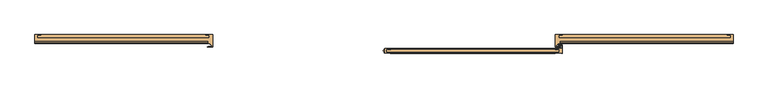
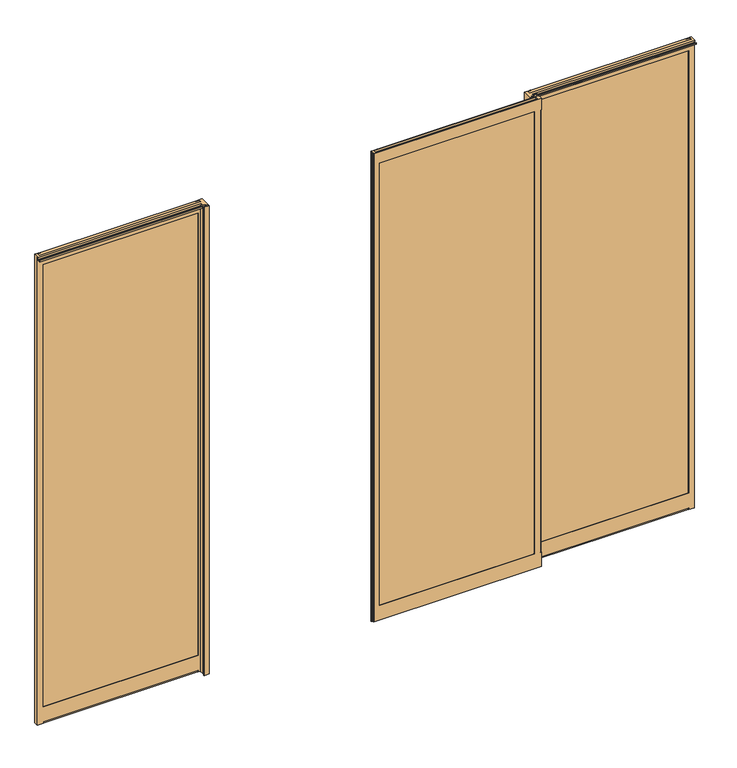
"""IFC4 building model written with IfcOpenShell, lengths in millimetres: door geometry, Otomatik Kapı-Çift Kanat : Otomatik Kapı - Çift Kanat - 150-220."""

from ifc_helpers import new_model, si_unit, point, frame, frame_2d, origin, place, context, project, spatial, polyline, circle_curve, trimmed, segment, composite_curve, outline, extrude, source, transform, mapped, element, save
from ifc_brep_helpers import plane_surface, cylinder_surface, revolved_surface, advanced_brep


def door_0aad8b15(model_context):
    return source(origin(), model_context, "Body", "SolidModel", [
        advanced_brep(
        [(1455.0015, 82.5, 0.0), (1480.0, 82.5, 0.0), (1480.0, 62.5, 0.0), (1455.0015331, 62.5, 0.0), (1455.0015331, 64.5000235, 0.0), (755.8014669, 64.5000827, 0.0), (755.8014669, 62.5, 0.0), (745.7999735, 62.5, 0.0), (745.7999735, 44.6000769, 0.0), (735.7999977, 44.6000769, 0.0), (735.7999977, 41.4071569, 0.0), (730.5928913, 36.2000504, 0.0), (727.8, 36.2000504, 0.0), (727.8, 33.1000319, 0.0), (744.8010861, 33.1000319, 0.0), (748.8010782, 30.7906337, 0.0), (748.8010782, 29.5000369, 0.0), (725.8, 29.5000369, 0.0), (725.8, 82.5, 0.0), (755.8015, 82.5, 0.0), (755.8015, 80.4999804, 0.0), (1455.0015, 80.5006675, 0.0), (1455.0015331, 62.5000013, 8.0), (1455.0015331, 64.5000261, 8.0), (1455.0015331, 64.500725, 2186.5000009), (1455.0015331, 64.5000485, 77.9996358), (1455.0015331, 62.500013, 77.9996641), (1455.0015331, 62.5003644, 2186.5000009), (1470.0015, 80.5007455, 62.9982401), (1470.0015, 64.5000436, 62.9982401), (1470.0015, 64.500725, 2201.5013187), (1470.0015, 80.5033922, 2201.5013187), (1470.0015, 80.5006675, 2232.0), (1470.0015, 80.5006675, 2230.5000015), (1470.0015, 69.0003591, 2230.5000015), (1470.0015, 67.5003602, 2232.0003428), (1455.0015, 80.5006675, 8.0), (1455.0015, 82.5000001, 8.0), (1455.0015, 82.5, 2232.0), (1455.0015, 82.5000175, 2230.5000015), (1455.0015, 80.5006675, 2230.5000015), (1455.0015, 80.5006675, 2232.0), (1455.0015, 82.5000175, 2186.500003), (1455.0015, 82.5000006, 77.9999376), (1455.0015, 80.5007647, 77.9999379), (1455.0015, 80.5033922, 2186.500003), (755.8015, 82.5000001, 8.0), (755.8015, 80.4999929, 8.0), (755.8015, 80.4999804, 2232.0), (755.8015, 80.4999804, 2230.5000015), (755.8015, 82.5000175, 2230.5000015), (755.8015, 82.5, 2232.0), (755.8015, 80.5033922, 2186.500003), (755.8015, 80.5001021, 77.9999379), (755.8015, 82.5000006, 77.9999376), (755.8015, 82.5000175, 2186.500003), (740.8, 64.500101, 62.9982401), (740.8, 80.500078, 62.9982401), (740.8, 80.5033922, 2201.5013187), (740.8, 64.500725, 2201.5013187), (740.8, 67.5003602, 2232.0003428), (740.8, 69.0003591, 2230.5000015), (740.8, 80.4999804, 2230.5000015), (740.8, 80.4999804, 2232.0), (755.8014669, 64.4996122, 8.0), (755.8014669, 62.5000013, 8.0), (755.8014669, 62.5003644, 2186.5000009), (755.8014669, 62.500013, 77.9996641), (755.8014669, 64.5001056, 77.9996358), (755.8014669, 64.500725, 2186.5000009), (745.7999735, 62.5003644, 2229.5000006), (745.7999735, 58.0999951, 2229.5000006), (745.7999735, 58.0999951, 2222.0024373), (745.7999735, 54.5998653, 2218.4999998), (745.7999735, 44.9999957, 2218.4999987), (745.7999735, 44.9999957, 2223.9999987), (745.7999735, 46.9999957, 2223.9999987), (745.7999735, 46.9999957, 2220.9999989), (745.7999735, 54.5999076, 2220.9999989), (745.7999735, 55.6000809, 2222.0001307), (745.7999735, 55.6000809, 2232.0003428), (745.7999735, 44.6000769, 2232.0), (735.7999977, 44.6000769, 2232.0), (725.8, 29.5000369, 2232.0), (748.8010782, 29.5000369, 2232.0), (1480.0, 82.5, 2232.0), (1480.0, 55.6000809, 2232.0003428), (1480.0, 55.6000809, 2222.0001307), (1480.0, 54.5999076, 2220.9999572), (1480.0, 46.9999957, 2220.9999989), (1480.0, 46.9999957, 2223.9999987), (1480.0, 44.9999957, 2223.9999987), (1480.0, 44.9999957, 2218.4999987), (1480.0, 54.5998653, 2218.4999987), (1480.0, 58.0999951, 2222.0024373), (1480.0, 58.0999951, 2229.5000006), (1480.0, 62.5003644, 2229.5000006), (725.8, 82.5, 2232.0), (748.8010782, 30.7906337, 2232.0003428), (744.8010861, 33.1000319, 2232.0003428), (727.8, 33.1000319, 2232.0003428), (727.8, 36.2000504, 2232.0003428), (730.5928913, 36.2000504, 2232.0003428), (735.7999977, 41.4071569, 2232.0003428)],
        [
            (0, 1),
            (1, 2),
            (2, 3),
            (3, 4),
            (4, 5),
            (5, 6),
            (6, 7),
            (7, 8),
            (8, 9),
            (9, 10),
            (10, 11),
            (11, 12),
            (12, 13),
            (13, 14),
            (14, 15),
            (15, 16),
            (16, 17),
            (17, 18),
            (18, 19),
            (19, 20),
            (20, 21),
            (21, 0),
            (3, 22),
            (22, 23),
            (23, 4),
            (24, 25),
            (25, 26),
            (26, 27),
            (27, 24),
            (28, 29),
            (29, 30),
            (30, 31),
            (31, 28),
            (32, 33),
            (33, 34),
            (34, 35),
            (35, 32),
            (21, 36),
            (36, 37),
            (37, 0),
            (38, 39),
            (39, 40),
            (40, 41),
            (41, 38),
            (42, 43),
            (43, 44),
            (44, 45),
            (45, 42),
            (19, 46),
            (46, 47),
            (47, 20),
            (48, 49),
            (49, 50),
            (50, 51),
            (51, 48),
            (52, 53),
            (53, 54),
            (54, 55),
            (55, 52),
            (56, 57),
            (57, 58),
            (58, 59),
            (59, 56),
            (60, 61),
            (61, 62),
            (62, 63),
            (63, 60),
            (5, 64),
            (64, 65),
            (65, 6),
            (66, 67),
            (67, 68),
            (68, 69),
            (69, 66),
            (70, 71),
            (71, 72),
            (72, 73, circle_curve(frame((745.7999735, 54.5998649, 2222.0001307), z_axis=(-1.0, 0.0, 0.0), x_axis=(0.0, 0.0, 1.0)), 3.5001309)),
            (73, 74),
            (74, 75),
            (75, 76),
            (76, 77),
            (77, 78),
            (78, 79, circle_curve(frame((745.7999735, 54.5999075, 2222.0001307), z_axis=(1.0, 0.0, 0.0), x_axis=(0.0, 0.0, 1.0)), 1.0001735)),
            (79, 80),
            (80, 81),
            (81, 8),
            (7, 70),
            (82, 9),
            (81, 82),
            (83, 17),
            (16, 84),
            (84, 83),
            (45, 52),
            (55, 42),
            (30, 59),
            (58, 31),
            (27, 66),
            (69, 24),
            (25, 68),
            (67, 26),
            (56, 29),
            (28, 57),
            (43, 54),
            (53, 44),
            (1, 85),
            (85, 86),
            (86, 87),
            (87, 88, circle_curve(frame((1480.0, 54.5999075, 2222.0001307), z_axis=(-1.0, 0.0, 0.0), x_axis=(0.0, 0.0, 1.0)), 1.0001735)),
            (88, 89),
            (89, 90),
            (90, 91),
            (91, 92),
            (92, 93),
            (93, 94, circle_curve(frame((1480.0, 54.5998649, 2222.0001307), z_axis=(1.0, 0.0, 0.0), x_axis=(0.0, 0.0, 1.0)), 3.5001309)),
            (94, 95),
            (95, 96),
            (96, 2),
            (83, 97),
            (97, 18),
            (41, 32),
            (35, 60),
            (63, 48),
            (51, 97),
            (84, 98),
            (98, 99),
            (99, 100),
            (100, 101),
            (101, 102),
            (102, 103),
            (103, 82),
            (80, 86),
            (85, 38),
            (37, 46),
            (50, 39),
            (40, 33),
            (62, 49),
            (96, 70),
            (65, 22),
            (34, 61),
            (95, 71),
            (94, 72),
            (93, 73),
            (92, 74),
            (91, 75),
            (90, 76),
            (89, 77),
            (88, 78),
            (87, 79),
            (103, 10),
            (102, 11),
            (101, 12),
            (100, 13),
            (99, 14),
            (98, 15),
            (36, 47),
            (23, 64),
        ],
        [
            plane_surface(frame((1480.0, 82.5, 0.0), z_axis=(0.0, 0.0, -1.0), x_axis=(0.0, -1.0, 0.0))),
            plane_surface(frame((1455.0015331, 62.5, 2232.0), z_axis=(-1.0, 0.0, 0.0), x_axis=(0.0, 0.0, -1.0))),
            plane_surface(frame((1470.0015, 64.5000235, 2232.0), z_axis=(-1.0, 0.0, 0.0), x_axis=(0.0, 0.0, -1.0))),
            plane_surface(frame((1455.0015, 80.5006675, 2232.0), z_axis=(-1.0, 0.0, 0.0), x_axis=(0.0, 0.0, -1.0))),
            plane_surface(frame((755.8015, 82.5, 2232.0), z_axis=(1.0, 0.0, 0.0), x_axis=(0.0, 0.0, -1.0))),
            plane_surface(frame((740.8, 80.4999804, 2232.0), z_axis=(1.0, 0.0, 0.0), x_axis=(0.0, 0.0, -1.0))),
            plane_surface(frame((755.8014669, 64.5000827, 2232.0), z_axis=(1.0, 0.0, 0.0), x_axis=(0.0, 0.0, -1.0))),
            plane_surface(frame((745.7999735, 62.5, 2232.0), z_axis=(1.0, 0.0, 0.0), x_axis=(0.0, 0.0, -1.0))),
            plane_surface(frame((745.7999735, 44.6000769, 2232.0), z_axis=(0.0, -1.0, 0.0), x_axis=(0.0, 0.0, -1.0))),
            plane_surface(frame((748.8010782, 29.5000369, 2232.0), z_axis=(0.0, -1.0, 0.0), x_axis=(0.0, 0.0, -1.0))),
            plane_surface(frame((1480.0, 82.5000175, 2186.500003), z_axis=(0.0, 0.0, -1.0), x_axis=(-1.0, 0.0, 0.0))),
            plane_surface(frame((1480.0, 80.5033922, 2201.5013187), z_axis=(0.0, 0.0, -1.0), x_axis=(-1.0, 0.0, 0.0))),
            plane_surface(frame((1480.0, 64.500725, 2186.5000009), z_axis=(0.0, 0.0, -1.0), x_axis=(-1.0, 0.0, 0.0))),
            plane_surface(frame((1480.0, 62.5, 77.9996641), z_axis=(0.0, 1.4132729652639372e-05, 0.999999999900133), x_axis=(-1.0, 0.0, 0.0))),
            plane_surface(frame((1480.0, 64.5000235, 62.9982401), z_axis=(0.0, 0.0, 1.0), x_axis=(-1.0, 0.0, 0.0))),
            plane_surface(frame((1480.0, 80.5000985, 77.9999379), z_axis=(0.0, 1.674987849023181e-07, 0.999999999999986), x_axis=(-1.0, 0.0, 0.0))),
            plane_surface(frame((1480.0, 82.5, 2232.0), z_axis=(1.0, 0.0, 0.0), x_axis=(0.0, -1.0, 0.0))),
            plane_surface(frame((725.8, 82.5, 2232.0), z_axis=(-1.0, 0.0, 0.0), x_axis=(0.0, -1.0, 0.0))),
            plane_surface(frame((1480.0, 55.6000809, 2232.0003428), z_axis=(0.0, 0.0, 1.0), x_axis=(-1.0, 0.0, 0.0))),
            plane_surface(frame((1480.0, 82.5000175, 2230.5000015), z_axis=(0.0, 1.0, 0.0), x_axis=(-1.0, 0.0, 0.0))),
            plane_surface(frame((1480.0, 80.5033922, 2186.500003), z_axis=(0.0, -1.0, 0.0), x_axis=(-1.0, 0.0, 0.0))),
            plane_surface(frame((1480.0, 64.500725, 2201.5013187), z_axis=(0.0, 1.0, 0.0), x_axis=(-1.0, 0.0, 0.0))),
            plane_surface(frame((1480.0, 62.5003644, 2186.5000009), z_axis=(0.0, -1.0, 0.0), x_axis=(-1.0, 0.0, 0.0))),
            plane_surface(frame((1480.0, 67.5003602, 2232.0003428), z_axis=(0.0, 0.7071874732725993, 0.7070260798911995), x_axis=(-1.0, 0.0, 0.0))),
            plane_surface(frame((1480.0, 69.0003591, 2230.5000015), z_axis=(0.0, 0.0, 1.0), x_axis=(-1.0, 0.0, 0.0))),
            plane_surface(frame((1480.0, 62.5003644, 2229.5000006), z_axis=(0.0, 0.0, -1.0), x_axis=(-1.0, 0.0, 0.0))),
            plane_surface(frame((1480.0, 58.0999951, 2229.5000006), z_axis=(0.0, 1.0, 0.0), x_axis=(-1.0, 0.0, 0.0))),
            cylinder_surface(frame((1480.0, 54.5998649, 2222.0001307), z_axis=(1.0, 0.0, 0.0), x_axis=(0.0, 0.0, 1.0)), 3.5001309),
            plane_surface(frame((1480.0, 54.5998653, 2218.4999987), z_axis=(0.0, 0.0, -1.0), x_axis=(-1.0, 0.0, 0.0))),
            plane_surface(frame((1480.0, 44.9999957, 2218.4999987), z_axis=(0.0, -1.0, 0.0), x_axis=(-1.0, 0.0, 0.0))),
            plane_surface(frame((1480.0, 44.9999957, 2223.9999987), z_axis=(0.0, 0.0, 1.0), x_axis=(-1.0, 0.0, 0.0))),
            plane_surface(frame((1480.0, 46.9999957, 2223.9999987), z_axis=(0.0, 1.0, 0.0), x_axis=(-1.0, 0.0, 0.0))),
            plane_surface(frame((1480.0, 46.9999957, 2220.9999989), z_axis=(0.0, 0.0, 1.0), x_axis=(-1.0, 0.0, 0.0))),
            revolved_surface(polyline([(745.7999735, 54.5999075, 2223.0003042000003), (1480.0, 54.5999075, 2223.0003042000003)]), (1480.0, 54.5999075, 2222.0001307), (-1.0, 0.0, 0.0)),
            plane_surface(frame((1480.0, 55.6000809, 2222.0001307), z_axis=(0.0, -1.0, 0.0), x_axis=(-1.0, 0.0, 0.0))),
            plane_surface(frame((735.7999977, 44.6000769, 2232.0), z_axis=(1.0, 0.0, 0.0), x_axis=(0.0, 0.0, -1.0))),
            plane_surface(frame((735.7999977, 41.4071569, 2232.0), z_axis=(0.7071067811865539, -0.7071067811865412, 0.0), x_axis=(0.0, 0.0, -1.0))),
            plane_surface(frame((730.5928913, 36.2000504, 2232.0), z_axis=(0.0, -1.0, 0.0), x_axis=(0.0, 0.0, -1.0))),
            plane_surface(frame((727.8, 36.2000504, 2232.0), z_axis=(1.0, 0.0, 0.0), x_axis=(0.0, 0.0, -1.0))),
            plane_surface(frame((727.8, 33.1000319, 2232.0), z_axis=(0.0, 1.0, 0.0), x_axis=(0.0, 0.0, -1.0))),
            plane_surface(frame((744.8010861, 33.1000319, 2232.0), z_axis=(0.5000002758229711, 0.8660252445379135, 0.0), x_axis=(0.0, 0.0, -1.0))),
            plane_surface(frame((748.8010782, 30.7906337, 2232.0), z_axis=(1.0, 0.0, 0.0), x_axis=(0.0, 0.0, -1.0))),
            plane_surface(frame((1480.0, 82.4999928, 8.0), z_axis=(0.0, 0.0, -1.0), x_axis=(-1.0, 0.0, 0.0))),
            plane_surface(frame((1480.0, 80.5006675, 8.0), z_axis=(0.0, 1.0, 0.0), x_axis=(-1.0, 0.0, 0.0))),
            plane_surface(frame((1480.0, 64.4996122, 0.0), z_axis=(0.0, -1.0, 0.0), x_axis=(-1.0, 0.0, 0.0))),
            plane_surface(frame((1480.0, 64.4996122, 8.0), z_axis=(0.0, 0.0, -1.0), x_axis=(-1.0, 0.0, 0.0))),
        ],
        [
            (0, [[1, 2, 3, 4, 5, 6, 7, 8, 9, 10, 11, 12, 13, 14, 15, 16, 17, 18, 19, 20, 21, 22]]),
            (1, [[23, 24, 25, -4]]),
            (1, [[26, 27, 28, 29]]),
            (2, [[30, 31, 32, 33]]),
            (2, [[34, 35, 36, 37]]),
            (3, [[38, 39, 40, -22]]),
            (3, [[41, 42, 43, 44]]),
            (3, [[45, 46, 47, 48]]),
            (4, [[49, 50, 51, -20]]),
            (4, [[52, 53, 54, 55]]),
            (4, [[56, 57, 58, 59]]),
            (5, [[60, 61, 62, 63]]),
            (5, [[64, 65, 66, 67]]),
            (6, [[68, 69, 70, -6]]),
            (6, [[71, 72, 73, 74]]),
            (7, [[75, 76, 77, 78, 79, 80, 81, 82, 83, 84, 85, 86, -8, 87]]),
            (8, [[88, -9, -86, 89]]),
            (9, [[90, -17, 91, 92]]),
            (10, [[93, -59, 94, -48]]),
            (11, [[95, -62, 96, -32]]),
            (12, [[97, -74, 98, -29]]),
            (13, [[-27, 99, -72, 100]]),
            (14, [[-60, 101, -30, 102]]),
            (15, [[-46, 103, -57, 104]]),
            (16, [[105, 106, 107, 108, 109, 110, 111, 112, 113, 114, 115, 116, 117, -2]]),
            (17, [[118, 119, -18, -90]]),
            (18, [[-44, 120, -37, 121, -67, 122, -55, 123, -118, -92, 124, 125, 126, 127, 128, 129, 130, -89, -85, 131, -106, 132]]),
            (19, [[-105, -1, -40, 133, -49, -19, -119, -123, -54, 134, -41, -132], [-94, -58, -103, -45]]),
            (20, [[-43, 135, -34, -120]]),
            (20, [[-66, 136, -52, -122]]),
            (20, [[-61, -102, -33, -96], [-47, -104, -56, -93]]),
            (21, [[-31, -101, -63, -95], [-73, -99, -26, -98]]),
            (22, [[-117, 137, -87, -7, -70, 138, -23, -3], [-97, -28, -100, -71]]),
            (23, [[139, -64, -121, -36]]),
            (24, [[-135, -42, -134, -53, -136, -65, -139, -35]]),
            (25, [[140, -75, -137, -116]]),
            (26, [[141, -76, -140, -115]]),
            (27, [[142, -77, -141, -114]]),
            (28, [[143, -78, -142, -113]]),
            (29, [[144, -79, -143, -112]]),
            (30, [[145, -80, -144, -111]]),
            (31, [[146, -81, -145, -110]]),
            (32, [[147, -82, -146, -109]]),
            (33, [[148, -83, -147, -108]]),
            (34, [[-131, -84, -148, -107]]),
            (35, [[149, -10, -88, -130]]),
            (36, [[150, -11, -149, -129]]),
            (37, [[151, -12, -150, -128]]),
            (38, [[152, -13, -151, -127]]),
            (39, [[153, -14, -152, -126]]),
            (40, [[154, -15, -153, -125]]),
            (41, [[-91, -16, -154, -124]]),
            (42, [[-50, -133, -39, 155]]),
            (43, [[-51, -155, -38, -21]]),
            (44, [[-25, 156, -68, -5]]),
            (45, [[-69, -156, -24, -138]]),
        ],
    ),
        extrude(outline(polyline([(743.292088, 75.4999975), (1467.9612743, 75.4999975), (1467.9612743, 65.4999975), (743.292088, 65.4999975), (743.292088, 75.4999975)])), frame((0.0, 0.0, 70.0), z_axis=(0.0, 0.0, 1.0), x_axis=(1.0, 0.0, 0.0)), (0.0, 0.0, 1.0), 2130.0),
        advanced_brep(
        [(-1455.0015, 82.5, 0.0), (-1455.0015, 80.5006675, 0.0), (-755.8015, 80.5033922, 0.0), (-755.8015, 82.5, 0.0), (-725.8, 82.5, 0.0), (-725.8, 29.5000369, 0.0), (-748.8010782, 29.5000369, 0.0), (-748.8010782, 30.7906337, 0.0), (-744.8010861, 33.1000319, 0.0), (-727.8, 33.1000319, 0.0), (-727.8, 36.2000504, 0.0), (-730.5928913, 36.2000504, 0.0), (-735.7999977, 41.4071569, 0.0), (-735.7999977, 44.6000769, 0.0), (-745.7999735, 44.6000769, 0.0), (-745.7999735, 62.5, 0.0), (-755.8014669, 62.5, 0.0), (-755.8014669, 64.5000827, 0.0), (-1455.0015331, 64.500725, 0.0), (-1455.0015331, 62.5, 0.0), (-1480.0, 62.5, 0.0), (-1480.0, 82.5, 0.0), (-1455.0015331, 64.4996122, 8.0), (-1455.0015331, 62.5000013, 8.0), (-1455.0015331, 64.500725, 2186.5000009), (-1455.0015331, 62.5003644, 2186.5000009), (-1455.0015331, 62.500013, 77.9996641), (-1455.0015331, 64.5000485, 77.9996358), (-1470.0015, 80.5006675, 2232.0), (-1470.0015, 67.5003602, 2232.0003428), (-1470.0015, 69.0003591, 2230.5000015), (-1470.0015, 80.5006675, 2230.5000015), (-1470.0015, 80.5007455, 62.9982401), (-1470.0015, 80.5033922, 2201.5013187), (-1470.0015, 64.500725, 2201.5013187), (-1470.0015, 64.5000436, 62.9982401), (-1455.0015, 82.5000001, 8.0), (-1455.0015, 80.5006775, 8.0), (-1455.0015, 82.5000175, 2186.500003), (-1455.0015, 80.5033922, 2186.500003), (-1455.0015, 80.5007647, 77.9999379), (-1455.0015, 82.5000006, 77.9999376), (-1455.0015, 82.5, 2232.0), (-1455.0015, 80.5006675, 2232.0), (-1455.0015, 80.5006675, 2230.5000015), (-1455.0015, 82.5000175, 2230.5000015), (-755.8015, 80.5006675, 8.0), (-755.8015, 82.5000001, 8.0), (-755.8015, 80.5033922, 2186.500003), (-755.8015, 82.5000175, 2186.500003), (-755.8015, 82.5000006, 77.9999376), (-755.8015, 80.5001021, 77.9999379), (-755.8015, 80.4999804, 2232.0), (-755.8015, 82.5, 2232.0), (-755.8015, 82.5000175, 2230.5000015), (-755.8015, 80.4999804, 2230.5000015), (-740.8, 67.5003602, 2232.0003428), (-740.8, 80.4999804, 2232.0), (-740.8, 80.4999804, 2230.5000015), (-740.8, 69.0003591, 2230.5000015), (-740.8, 64.500101, 62.9982401), (-740.8, 64.500725, 2201.5013187), (-740.8, 80.5033922, 2201.5013187), (-740.8, 80.500078, 62.9982401), (-755.8014669, 62.5000013, 8.0), (-755.8014669, 64.500085, 8.0), (-755.8014669, 62.5003644, 2186.5000009), (-755.8014669, 64.500725, 2186.5000009), (-755.8014669, 64.5001056, 77.9996358), (-755.8014669, 62.500013, 77.9996641), (-745.7999735, 62.5003644, 2229.5000006), (-745.7999735, 44.6000769, 2232.0), (-745.7999735, 55.6000809, 2232.0003428), (-745.7999735, 55.6000809, 2222.0001307), (-745.7999735, 54.5999076, 2220.9999572), (-745.7999735, 46.9999957, 2220.9999989), (-745.7999735, 46.9999957, 2223.9999987), (-745.7999735, 44.9999957, 2223.9999987), (-745.7999735, 44.9999957, 2218.4999987), (-745.7999735, 54.5998653, 2218.4999987), (-745.7999735, 58.0999951, 2222.0024373), (-745.7999735, 58.0999951, 2229.5000006), (-735.7999977, 44.6000769, 2232.0), (-725.8, 29.5000369, 2232.0), (-748.8010782, 29.5000369, 2232.0), (-1480.0, 62.5003644, 2229.5000006), (-1480.0, 58.0999951, 2229.5000006), (-1480.0, 58.0999951, 2222.0024373), (-1480.0, 54.5998653, 2218.4999998), (-1480.0, 44.9999957, 2218.4999987), (-1480.0, 44.9999957, 2223.9999987), (-1480.0, 46.9999957, 2223.9999987), (-1480.0, 46.9999957, 2220.9999989), (-1480.0, 54.599865, 2220.9999989), (-1480.0, 55.6000809, 2222.0001307), (-1480.0, 55.6000809, 2232.0003428), (-1480.0, 82.5, 2232.0), (-725.8, 82.5, 2232.0), (-735.7999977, 41.4071569, 2232.0003428), (-730.5928913, 36.2000504, 2232.0003428), (-727.8, 36.2000504, 2232.0003428), (-727.8, 33.1000319, 2232.0003428), (-744.8010861, 33.1000319, 2232.0003428), (-748.8010782, 30.7906337, 2232.0003428)],
        [
            (0, 1),
            (1, 2),
            (2, 3),
            (3, 4),
            (4, 5),
            (5, 6),
            (6, 7),
            (7, 8),
            (8, 9),
            (9, 10),
            (10, 11),
            (11, 12),
            (12, 13),
            (13, 14),
            (14, 15),
            (15, 16),
            (16, 17),
            (17, 18),
            (18, 19),
            (19, 20),
            (20, 21),
            (21, 0),
            (18, 22),
            (22, 23),
            (23, 19),
            (24, 25),
            (25, 26),
            (26, 27),
            (27, 24),
            (28, 29),
            (29, 30),
            (30, 31),
            (31, 28),
            (32, 33),
            (33, 34),
            (34, 35),
            (35, 32),
            (0, 36),
            (36, 37),
            (37, 1),
            (38, 39),
            (39, 40),
            (40, 41),
            (41, 38),
            (42, 43),
            (43, 44),
            (44, 45),
            (45, 42),
            (2, 46),
            (46, 47),
            (47, 3),
            (48, 49),
            (49, 50),
            (50, 51),
            (51, 48),
            (52, 53),
            (53, 54),
            (54, 55),
            (55, 52),
            (56, 57),
            (57, 58),
            (58, 59),
            (59, 56),
            (60, 61),
            (61, 62),
            (62, 63),
            (63, 60),
            (16, 64),
            (64, 65),
            (65, 17),
            (66, 67),
            (67, 68),
            (68, 69),
            (69, 66),
            (70, 15),
            (14, 71),
            (71, 72),
            (72, 73),
            (73, 74, circle_curve(frame((-745.7999735, 54.5999075, 2222.0001307), z_axis=(-1.0, 0.0, 0.0), x_axis=(0.0, 0.0, 1.0)), 1.0001735)),
            (74, 75),
            (75, 76),
            (76, 77),
            (77, 78),
            (78, 79),
            (79, 80, circle_curve(frame((-745.7999735, 54.5998649, 2222.0001307), z_axis=(1.0, 0.0, 0.0), x_axis=(0.0, 0.0, 1.0)), 3.5001309)),
            (80, 81),
            (81, 70),
            (82, 71),
            (13, 82),
            (83, 84),
            (84, 6),
            (5, 83),
            (38, 49),
            (48, 39),
            (33, 62),
            (61, 34),
            (24, 67),
            (66, 25),
            (26, 69),
            (68, 27),
            (63, 32),
            (35, 60),
            (40, 51),
            (50, 41),
            (20, 85),
            (85, 86),
            (86, 87),
            (87, 88, circle_curve(frame((-1480.0, 54.5998649, 2222.0001307), z_axis=(-1.0, 0.0, 0.0), x_axis=(0.0, 0.0, 1.0)), 3.5001309)),
            (88, 89),
            (89, 90),
            (90, 91),
            (91, 92),
            (92, 93),
            (93, 94, circle_curve(frame((-1480.0, 54.5999075, 2222.0001307), z_axis=(1.0, 0.0, 0.0), x_axis=(0.0, 0.0, 1.0)), 1.0001735)),
            (94, 95),
            (95, 96),
            (96, 21),
            (4, 97),
            (97, 83),
            (42, 96),
            (95, 72),
            (82, 98),
            (98, 99),
            (99, 100),
            (100, 101),
            (101, 102),
            (102, 103),
            (103, 84),
            (97, 53),
            (52, 57),
            (56, 29),
            (28, 43),
            (45, 54),
            (47, 36),
            (55, 58),
            (31, 44),
            (23, 64),
            (70, 85),
            (59, 30),
            (81, 86),
            (80, 87),
            (79, 88),
            (78, 89),
            (77, 90),
            (76, 91),
            (75, 92),
            (74, 93),
            (73, 94),
            (12, 98),
            (11, 99),
            (10, 100),
            (9, 101),
            (8, 102),
            (7, 103),
            (46, 37),
            (65, 22),
        ],
        [
            plane_surface(frame((-1480.0, 82.5, 0.0), z_axis=(0.0, 0.0, -1.0), x_axis=(0.0, -1.0, 0.0))),
            plane_surface(frame((-1455.0015331, 62.5, 2232.0), z_axis=(1.0, 0.0, 0.0), x_axis=(0.0, 0.0, -1.0))),
            plane_surface(frame((-1470.0015, 64.5000235, 2232.0), z_axis=(1.0, 0.0, 0.0), x_axis=(0.0, 0.0, -1.0))),
            plane_surface(frame((-1455.0015, 80.5006675, 2232.0), z_axis=(1.0, 0.0, 0.0), x_axis=(0.0, 0.0, -1.0))),
            plane_surface(frame((-755.8015, 82.5, 2232.0), z_axis=(-1.0, 0.0, 0.0), x_axis=(0.0, 0.0, -1.0))),
            plane_surface(frame((-740.8, 80.4999804, 2232.0), z_axis=(-1.0, 0.0, 0.0), x_axis=(0.0, 0.0, -1.0))),
            plane_surface(frame((-755.8014669, 64.5000827, 2232.0), z_axis=(-1.0, 0.0, 0.0), x_axis=(0.0, 0.0, -1.0))),
            plane_surface(frame((-745.7999735, 62.5, 2232.0), z_axis=(-1.0, 0.0, 0.0), x_axis=(0.0, 0.0, -1.0))),
            plane_surface(frame((-745.7999735, 44.6000769, 2232.0), z_axis=(0.0, -1.0, 0.0), x_axis=(0.0, 0.0, -1.0))),
            plane_surface(frame((-748.8010782, 29.5000369, 2232.0), z_axis=(0.0, -1.0, 0.0), x_axis=(0.0, 0.0, -1.0))),
            plane_surface(frame((-1480.0, 82.5000175, 2186.500003), z_axis=(0.0, 0.0, -1.0), x_axis=(1.0, 0.0, 0.0))),
            plane_surface(frame((-1480.0, 80.5033922, 2201.5013187), z_axis=(0.0, 0.0, -1.0), x_axis=(1.0, 0.0, 0.0))),
            plane_surface(frame((-1480.0, 64.500725, 2186.5000009), z_axis=(0.0, 0.0, -1.0), x_axis=(1.0, 0.0, 0.0))),
            plane_surface(frame((-1480.0, 62.5, 77.9996641), z_axis=(0.0, 1.4132729652639372e-05, 0.999999999900133), x_axis=(1.0, 0.0, 0.0))),
            plane_surface(frame((-1480.0, 64.5000235, 62.9982401), z_axis=(0.0, 0.0, 1.0), x_axis=(1.0, 0.0, 0.0))),
            plane_surface(frame((-1480.0, 80.5000985, 77.9999379), z_axis=(0.0, 1.674987849023181e-07, 0.999999999999986), x_axis=(1.0, 0.0, 0.0))),
            plane_surface(frame((-1480.0, 82.5, 2232.0), z_axis=(-1.0, 0.0, 0.0), x_axis=(0.0, -1.0, 0.0))),
            plane_surface(frame((-725.8, 82.5, 2232.0), z_axis=(1.0, 0.0, 0.0), x_axis=(0.0, -1.0, 0.0))),
            plane_surface(frame((-1480.0, 55.6000809, 2232.0003428), z_axis=(0.0, 0.0, 1.0), x_axis=(1.0, 0.0, 0.0))),
            plane_surface(frame((-1480.0, 82.5000175, 2230.5000015), z_axis=(0.0, 1.0, 0.0), x_axis=(1.0, 0.0, 0.0))),
            plane_surface(frame((-1480.0, 80.5033922, 2186.500003), z_axis=(0.0, -1.0, 0.0), x_axis=(1.0, 0.0, 0.0))),
            plane_surface(frame((-1480.0, 64.500725, 2201.5013187), z_axis=(0.0, 1.0, 0.0), x_axis=(1.0, 0.0, 0.0))),
            plane_surface(frame((-1480.0, 62.5003644, 2186.5000009), z_axis=(0.0, -1.0, 0.0), x_axis=(1.0, 0.0, 0.0))),
            plane_surface(frame((-1480.0, 67.5003602, 2232.0003428), z_axis=(0.0, 0.7071874732725993, 0.7070260798911995), x_axis=(1.0, 0.0, 0.0))),
            plane_surface(frame((-1480.0, 69.0003591, 2230.5000015), z_axis=(0.0, 0.0, 1.0), x_axis=(1.0, 0.0, 0.0))),
            plane_surface(frame((-1480.0, 62.5003644, 2229.5000006), z_axis=(0.0, 0.0, -1.0), x_axis=(1.0, 0.0, 0.0))),
            plane_surface(frame((-1480.0, 58.0999951, 2229.5000006), z_axis=(0.0, 1.0, 0.0), x_axis=(1.0, 0.0, 0.0))),
            cylinder_surface(frame((-1480.0, 54.5998649, 2222.0001307), z_axis=(-1.0, 0.0, 0.0), x_axis=(0.0, 0.0, 1.0)), 3.5001309),
            plane_surface(frame((-1480.0, 54.5998653, 2218.4999987), z_axis=(0.0, 0.0, -1.0), x_axis=(1.0, 0.0, 0.0))),
            plane_surface(frame((-1480.0, 44.9999957, 2218.4999987), z_axis=(0.0, -1.0, 0.0), x_axis=(1.0, 0.0, 0.0))),
            plane_surface(frame((-1480.0, 44.9999957, 2223.9999987), z_axis=(0.0, 0.0, 1.0), x_axis=(1.0, 0.0, 0.0))),
            plane_surface(frame((-1480.0, 46.9999957, 2223.9999987), z_axis=(0.0, 1.0, 0.0), x_axis=(1.0, 0.0, 0.0))),
            plane_surface(frame((-1480.0, 46.9999957, 2220.9999989), z_axis=(0.0, 0.0, 1.0), x_axis=(1.0, 0.0, 0.0))),
            revolved_surface(polyline([(-745.7999735, 54.5999075, 2223.0003042000003), (-1480.0, 54.5999075, 2223.0003042000003)]), (-1480.0, 54.5999075, 2222.0001307), (1.0, 0.0, 0.0)),
            plane_surface(frame((-1480.0, 55.6000809, 2222.0001307), z_axis=(0.0, -1.0, 0.0), x_axis=(1.0, 0.0, 0.0))),
            plane_surface(frame((-735.7999977, 44.6000769, 2232.0), z_axis=(-1.0, 0.0, 0.0), x_axis=(0.0, 0.0, -1.0))),
            plane_surface(frame((-735.7999977, 41.4071569, 2232.0), z_axis=(-0.7071067811865539, -0.7071067811865412, 0.0), x_axis=(0.0, 0.0, -1.0))),
            plane_surface(frame((-730.5928913, 36.2000504, 2232.0), z_axis=(0.0, -1.0, 0.0), x_axis=(0.0, 0.0, -1.0))),
            plane_surface(frame((-727.8, 36.2000504, 2232.0), z_axis=(-1.0, 0.0, 0.0), x_axis=(0.0, 0.0, -1.0))),
            plane_surface(frame((-727.8, 33.1000319, 2232.0), z_axis=(0.0, 1.0, 0.0), x_axis=(0.0, 0.0, -1.0))),
            plane_surface(frame((-744.8010861, 33.1000319, 2232.0), z_axis=(-0.5000002758229711, 0.8660252445379135, 0.0), x_axis=(0.0, 0.0, -1.0))),
            plane_surface(frame((-748.8010782, 30.7906337, 2232.0), z_axis=(-1.0, 0.0, 0.0), x_axis=(0.0, 0.0, -1.0))),
            plane_surface(frame((-1480.0, 82.4999928, 8.0), z_axis=(0.0, 0.0, -1.0), x_axis=(1.0, 0.0, 0.0))),
            plane_surface(frame((-1480.0, 80.5006675, 8.0), z_axis=(0.0, 1.0, 0.0), x_axis=(1.0, 0.0, 0.0))),
            plane_surface(frame((-1480.0, 64.4996122, 0.0), z_axis=(0.0, -1.0, 0.0), x_axis=(1.0, 0.0, 0.0))),
            plane_surface(frame((-1480.0, 64.4996122, 8.0), z_axis=(0.0, 0.0, -1.0), x_axis=(1.0, 0.0, 0.0))),
        ],
        [
            (0, [[1, 2, 3, 4, 5, 6, 7, 8, 9, 10, 11, 12, 13, 14, 15, 16, 17, 18, 19, 20, 21, 22]]),
            (1, [[-19, 23, 24, 25]]),
            (1, [[26, 27, 28, 29]]),
            (2, [[30, 31, 32, 33]]),
            (2, [[34, 35, 36, 37]]),
            (3, [[-1, 38, 39, 40]]),
            (3, [[41, 42, 43, 44]]),
            (3, [[45, 46, 47, 48]]),
            (4, [[-3, 49, 50, 51]]),
            (4, [[52, 53, 54, 55]]),
            (4, [[56, 57, 58, 59]]),
            (5, [[60, 61, 62, 63]]),
            (5, [[64, 65, 66, 67]]),
            (6, [[-17, 68, 69, 70]]),
            (6, [[71, 72, 73, 74]]),
            (7, [[75, -15, 76, 77, 78, 79, 80, 81, 82, 83, 84, 85, 86, 87]]),
            (8, [[88, -76, -14, 89]]),
            (9, [[90, 91, -6, 92]]),
            (10, [[-41, 93, -52, 94]]),
            (11, [[-35, 95, -65, 96]]),
            (12, [[-26, 97, -71, 98]]),
            (13, [[99, -73, 100, -28]]),
            (14, [[101, -37, 102, -67]]),
            (15, [[103, -54, 104, -43]]),
            (16, [[-21, 105, 106, 107, 108, 109, 110, 111, 112, 113, 114, 115, 116, 117]]),
            (17, [[-92, -5, 118, 119]]),
            (18, [[120, -116, 121, -77, -88, 122, 123, 124, 125, 126, 127, 128, -90, -119, 129, -56, 130, -60, 131, -30, 132, -45]]),
            (19, [[-120, -48, 133, -57, -129, -118, -4, -51, 134, -38, -22, -117], [-44, -104, -53, -93]]),
            (20, [[-95, -34, -101, -66], [-94, -55, -103, -42]]),
            (20, [[-130, -59, 135, -61]]),
            (20, [[-132, -33, 136, -46]]),
            (21, [[-96, -64, -102, -36], [-97, -29, -100, -72]]),
            (22, [[-20, -25, 137, -68, -16, -75, 138, -105], [-74, -99, -27, -98]]),
            (23, [[-31, -131, -63, 139]]),
            (24, [[-32, -139, -62, -135, -58, -133, -47, -136]]),
            (25, [[-106, -138, -87, 140]]),
            (26, [[-107, -140, -86, 141]]),
            (27, [[-108, -141, -85, 142]]),
            (28, [[-109, -142, -84, 143]]),
            (29, [[-110, -143, -83, 144]]),
            (30, [[-111, -144, -82, 145]]),
            (31, [[-112, -145, -81, 146]]),
            (32, [[-113, -146, -80, 147]]),
            (33, [[-114, -147, -79, 148]]),
            (34, [[-115, -148, -78, -121]]),
            (35, [[-122, -89, -13, 149]]),
            (36, [[-123, -149, -12, 150]]),
            (37, [[-124, -150, -11, 151]]),
            (38, [[-125, -151, -10, 152]]),
            (39, [[-126, -152, -9, 153]]),
            (40, [[-127, -153, -8, 154]]),
            (41, [[-128, -154, -7, -91]]),
            (42, [[155, -39, -134, -50]]),
            (43, [[-2, -40, -155, -49]]),
            (44, [[-18, -70, 156, -23]]),
            (45, [[-137, -24, -156, -69]]),
        ],
    ),
        extrude(outline(polyline([(-743.292088, 75.4999975), (-743.292088, 65.4999975), (-1467.9612743, 65.4999975), (-1467.9612743, 75.4999975), (-743.292088, 75.4999975)])), frame((0.0, 0.0, 70.0), z_axis=(0.0, 0.0, 1.0), x_axis=(1.0, 0.0, 0.0)), (0.0, 0.0, 1.0), 2130.0),
        advanced_brep(
        [(756.7, 35.2330503, 8.0000212), (756.7, 3.7, 8.0000212), (2.5, 3.7, 8.0000212), (2.5, 23.6999918, 8.0000212), (754.7, 23.7, 8.0000212), (754.7, 35.1861454, 8.0000212), (753.6861454, 36.2, 8.0000212), (741.69925, 36.2, 8.0000212), (741.69925, 38.2, 8.0000212), (753.7330503, 38.2, 8.0000212), (741.69925, 10.2025832, 8.0000212), (741.69925, 17.1998167, 8.0000212), (12.4985, 17.1998167, 8.0000212), (12.4985, 10.2025832, 8.0000212), (754.7, 23.7, 2241.0), (2.5, 23.7, 2241.0), (2.5, 3.7, 2241.0), (756.7, 3.7, 2241.0), (756.7, 35.2330503, 2241.0), (753.7330503, 38.2, 2241.0), (741.69925, 38.2, 2241.0), (741.69925, 36.2, 2241.0), (753.6861454, 36.2, 2241.0), (754.7, 35.1861454, 2241.0), (741.69925, 18.701, 2241.0), (741.69925, 8.699, 2241.0), (12.4985, 8.699, 2241.0), (12.4985, 18.701, 2241.0), (756.7, 3.7, 2186.0007973), (756.7, 5.7, 2186.0007973), (756.7, 5.7, 2201.0007973), (756.7, 6.760542, 2201.0007973), (756.7, 6.760542, 62.9982446), (756.7, 5.7, 62.9982446), (756.7, 5.7, 78.000055), (756.7, 3.7, 78.000055), (726.6862373, 23.7, 2186.0004744), (726.6862373, 23.7, 77.9999799), (726.6862373, 21.7006279, 77.9999799), (726.6862373, 21.7006279, 2186.0004744), (741.69925, 21.7006279, 2201.0007973), (12.4985, 21.7006279, 2201.0007973), (12.4985, 21.7006279, 62.9982446), (741.69925, 21.7006279, 62.9982446), (27.4985, 21.7006279, 77.9999799), (27.4985, 21.7006279, 2186.0004744), (741.69925, 5.7, 62.9982446), (741.69925, 5.7, 2201.0007973), (741.69925, 18.701, 2232.5), (741.69925, 8.699, 2232.5), (741.69925, 10.2025832, 33.4998483), (741.69925, 17.1998167, 33.4998483), (756.5103756, 5.7, 2186.0007973), (756.5103756, 5.7, 2201.0007973), (756.5103756, 5.7, 62.9982446), (756.5103756, 5.7, 78.000055), (12.4985, 5.7, 62.9982446), (12.4985, 5.7, 2201.0007973), (726.6985, 5.7, 2186.0007973), (27.4985, 5.7, 2186.0007973), (27.4985, 5.7, 78.000055), (726.6985, 5.7, 78.000055), (726.6985, 3.7, 78.000055), (726.6985, 3.7, 2186.0007973), (753.639458, 3.7, 78.000055), (753.639458, 3.7, 2186.0007973), (27.4985, 3.7, 78.000055), (27.4985, 3.7, 2186.0007973), (27.4985, 23.7, 2186.0004744), (27.4985, 23.7, 77.9999799), (12.4985, 8.699, 2232.5), (12.4985, 18.701, 2232.5), (12.4985, 17.1998167, 33.4998483), (12.4985, 10.2025832, 33.4998483)],
        [
            (0, 1),
            (1, 2),
            (2, 3),
            (3, 4),
            (4, 5),
            (5, 6, circle_curve(frame((753.6861454, 35.1861454, 8.0000212), z_axis=(0.0, 0.0, 1.0), x_axis=(1.0, 0.0, 0.0)), 1.0138546)),
            (6, 7),
            (7, 8),
            (8, 9),
            (9, 0, circle_curve(frame((753.7330503, 35.2330503, 8.0000212), z_axis=(0.0, 0.0, -1.0), x_axis=(1.0, 0.0, 0.0)), 2.9669497)),
            (10, 11),
            (11, 12),
            (12, 13),
            (13, 10),
            (14, 15),
            (15, 16),
            (16, 17),
            (17, 18),
            (18, 19, circle_curve(frame((753.7330503, 35.2330503, 2241.0), z_axis=(0.0, 0.0, 1.0), x_axis=(1.0, 0.0, 0.0)), 2.9669497)),
            (19, 20),
            (20, 21),
            (21, 22),
            (22, 23, circle_curve(frame((753.6861454, 35.1861454, 2241.0), z_axis=(0.0, 0.0, -1.0), x_axis=(1.0, 0.0, 0.0)), 1.0138546)),
            (23, 14),
            (24, 25),
            (25, 26),
            (26, 27),
            (27, 24),
            (17, 28),
            (28, 29),
            (29, 30),
            (30, 31),
            (31, 32),
            (32, 33),
            (33, 34),
            (34, 35),
            (35, 1),
            (0, 18),
            (8, 20),
            (19, 9),
            (7, 21),
            (36, 37),
            (37, 38),
            (38, 39),
            (39, 36),
            (40, 41),
            (41, 42),
            (42, 43),
            (43, 40),
            (38, 44),
            (44, 45),
            (45, 39),
            (43, 46),
            (46, 47),
            (47, 40),
            (24, 48),
            (48, 49),
            (49, 25),
            (10, 50),
            (50, 51),
            (51, 11),
            (29, 52),
            (52, 53),
            (53, 30),
            (33, 54),
            (54, 55),
            (55, 34),
            (46, 56),
            (56, 57),
            (57, 47),
            (58, 59),
            (59, 60),
            (60, 61),
            (61, 58),
            (61, 62),
            (62, 63),
            (63, 58),
            (16, 2),
            (35, 64),
            (64, 65),
            (65, 28),
            (62, 66),
            (66, 67),
            (67, 63),
            (14, 4),
            (3, 15),
            (36, 68),
            (68, 69),
            (69, 37),
            (6, 22),
            (23, 5),
            (52, 65, circle_curve(frame((753.639458, 6.760542, 2186.0007973), z_axis=(0.0, 0.0, -1.0), x_axis=(1.0, 0.0, 0.0)), 3.060542)),
            (64, 55, circle_curve(frame((753.639458, 6.760542, 78.000055), z_axis=(0.0, 0.0, 1.0), x_axis=(1.0, 0.0, 0.0)), 3.060542)),
            (54, 32, circle_curve(frame((753.639458, 6.760542, 62.9982446), z_axis=(0.0, 0.0, 1.0), x_axis=(1.0, 0.0, 0.0)), 3.060542)),
            (31, 53, circle_curve(frame((753.639458, 6.760542, 2201.0007973), z_axis=(0.0, 0.0, -1.0), x_axis=(1.0, 0.0, 0.0)), 3.060542)),
            (49, 70),
            (70, 26),
            (48, 71),
            (71, 70),
            (27, 71),
            (45, 68),
            (57, 41),
            (67, 59),
            (60, 66),
            (42, 56),
            (69, 44),
            (51, 72),
            (72, 12),
            (50, 73),
            (73, 72),
            (13, 73),
        ],
        [
            plane_surface(frame((756.7, 23.7, 8.0000212), z_axis=(0.0, 0.0, -1.0), x_axis=(0.0, -1.0, 0.0))),
            plane_surface(frame((756.7, 23.7, 2241.0), z_axis=(0.0, 0.0, 1.0), x_axis=(0.0, -1.0, 0.0))),
            plane_surface(frame((756.7, 6.760542, 8.0000212), z_axis=(1.0, 0.0, 0.0), x_axis=(0.0, 0.0, 1.0))),
            plane_surface(frame((753.7330503, 38.2, 8.0000212), z_axis=(0.0, 1.0, 0.0), x_axis=(0.0, 0.0, 1.0))),
            plane_surface(frame((741.69925, 38.2, 8.0000212), z_axis=(-1.0, 0.0, 0.0), x_axis=(0.0, 0.0, 1.0))),
            plane_surface(frame((726.6862373, 23.7, 8.0000212), z_axis=(-1.0, 0.0, 0.0), x_axis=(0.0, 0.0, 1.0))),
            plane_surface(frame((726.6862373, 21.7006279, 8.0000212), z_axis=(0.0, -1.0, 0.0), x_axis=(0.0, 0.0, 1.0))),
            plane_surface(frame((741.69925, 21.7006279, 8.0000212), z_axis=(-1.0, 0.0, 0.0), x_axis=(0.0, 0.0, 1.0))),
            plane_surface(frame((741.69925, 5.7, 8.0000212), z_axis=(0.0, 1.0, 0.0), x_axis=(0.0, 0.0, 1.0))),
            plane_surface(frame((726.6985, 5.7, 8.0000212), z_axis=(-1.0, 0.0, 0.0), x_axis=(0.0, 0.0, 1.0))),
            plane_surface(frame((726.6985, 3.7, 8.0000212), z_axis=(0.0, -1.0, 0.0), x_axis=(0.0, 0.0, 1.0))),
            plane_surface(frame((754.7, 23.7, 8.0000212), z_axis=(0.0, 1.0, 0.0), x_axis=(0.0, 0.0, 1.0))),
            plane_surface(frame((741.69925, 36.2, 8.0000212), z_axis=(0.0, -1.0, 0.0), x_axis=(0.0, 0.0, 1.0))),
            plane_surface(frame((754.7, 35.1861454, 8.0000212), z_axis=(-1.0, 0.0, 0.0), x_axis=(0.0, 0.0, 1.0))),
            cylinder_surface(frame((753.639458, 6.760542, 8.0000212), z_axis=(0.0, 0.0, -1.0), x_axis=(1.0, 0.0, 0.0)), 3.060542),
            cylinder_surface(frame((753.7330503, 35.2330503, 8.0000212), z_axis=(0.0, 0.0, -1.0), x_axis=(1.0, 0.0, 0.0)), 2.9669497),
            revolved_surface(polyline([(754.6999999999999, 35.1861454, 2241.0), (754.6999999999999, 35.1861454, 8.0000212)]), (753.6861454, 35.1861454, 8.0000212), (0.0, 0.0, 1.0)),
            plane_surface(frame((2.5, 23.7, 2241.0), z_axis=(-1.0, 0.0, 0.0), x_axis=(0.0, -1.0, 0.0))),
            plane_surface(frame((756.7, 8.699, 2241.0), z_axis=(0.0, 1.0, 0.0), x_axis=(-1.0, 0.0, 0.0))),
            plane_surface(frame((756.7, 8.699, 2232.5), z_axis=(0.0, 0.0, 1.0), x_axis=(-1.0, 0.0, 0.0))),
            plane_surface(frame((756.7, 18.701, 2232.5), z_axis=(0.0, -1.0, 0.0), x_axis=(-1.0, 0.0, 0.0))),
            plane_surface(frame((756.7, 23.7, 2186.0004744), z_axis=(0.0, 0.0, -1.0), x_axis=(-1.0, 0.0, 0.0))),
            plane_surface(frame((756.7, 21.7, 2201.0007973), z_axis=(0.0, 0.0, -1.0), x_axis=(-1.0, 0.0, 0.0))),
            plane_surface(frame((756.7, 5.7, 2186.0007973), z_axis=(0.0, 0.0, -1.0), x_axis=(-1.0, 0.0, 0.0))),
            plane_surface(frame((756.7, 3.7, 78.000055), z_axis=(0.0, 0.0, 1.0), x_axis=(-1.0, 0.0, 0.0))),
            plane_surface(frame((756.7, 5.7, 62.9982446), z_axis=(0.0, 0.0, 1.0), x_axis=(-1.0, 0.0, 0.0))),
            plane_surface(frame((756.7, 21.6999777, 77.9999799), z_axis=(0.0, 0.0, 1.0), x_axis=(-1.0, 0.0, 0.0))),
            plane_surface(frame((756.7, 17.1998167, 8.0000212), z_axis=(0.0, -1.0, 0.0), x_axis=(-1.0, 0.0, 0.0))),
            plane_surface(frame((756.7, 17.1998167, 33.4998483), z_axis=(0.0, 0.0, -1.0), x_axis=(-1.0, 0.0, 0.0))),
            plane_surface(frame((756.7, 10.2025832, 33.4998483), z_axis=(0.0, 1.0, 0.0), x_axis=(-1.0, 0.0, 0.0))),
            plane_surface(frame((27.4985, 3.7, 8.0000212), z_axis=(1.0, 0.0, 0.0), x_axis=(0.0, 0.0, 1.0))),
            plane_surface(frame((12.4985, 5.7, 8.0000212), z_axis=(1.0, 0.0, 0.0), x_axis=(0.0, 0.0, 1.0))),
            plane_surface(frame((27.4985, 21.7, 8.0000212), z_axis=(1.0, 0.0, 0.0), x_axis=(0.0, 0.0, 1.0))),
        ],
        [
            (0, [[1, 2, 3, 4, 5, 6, 7, 8, 9, 10], [11, 12, 13, 14]]),
            (1, [[15, 16, 17, 18, 19, 20, 21, 22, 23, 24], [25, 26, 27, 28]]),
            (2, [[-18, 29, 30, 31, 32, 33, 34, 35, 36, 37, -1, 38]]),
            (3, [[39, -20, 40, -9]]),
            (4, [[41, -21, -39, -8]]),
            (5, [[42, 43, 44, 45]]),
            (6, [[46, 47, 48, 49], [50, 51, 52, -44]]),
            (7, [[-49, 53, 54, 55]]),
            (7, [[56, 57, 58, -25]]),
            (7, [[59, 60, 61, -11]]),
            (8, [[62, 63, 64, -31]]),
            (8, [[65, 66, 67, -35]]),
            (8, [[68, 69, 70, -54], [71, 72, 73, 74]]),
            (9, [[-74, 75, 76, 77]]),
            (10, [[78, -2, -37, 79, 80, 81, -29, -17], [-76, 82, 83, 84]]),
            (11, [[85, -4, 86, -15], [-42, 87, 88, 89]]),
            (12, [[90, -22, -41, -7]]),
            (13, [[-85, -24, 91, -5]]),
            (14, [[-63, 92, -80, 93, -66, 94, -33, 95]]),
            (15, [[-40, -19, -38, -10]]),
            (16, [[-91, -23, -90, -6]]),
            (17, [[-16, -86, -3, -78]]),
            (18, [[96, 97, -26, -58]]),
            (19, [[98, 99, -96, -57]]),
            (20, [[-28, 100, -98, -56]]),
            (21, [[-52, 101, -87, -45]]),
            (22, [[-64, -95, -32]]),
            (22, [[102, -46, -55, -70]]),
            (23, [[-84, 103, -71, -77]]),
            (23, [[-81, -92, -62, -30]]),
            (24, [[-67, -93, -79, -36]]),
            (24, [[-73, 104, -82, -75]]),
            (25, [[-94, -65, -34]]),
            (25, [[105, -68, -53, -48]]),
            (26, [[-89, 106, -50, -43]]),
            (27, [[107, 108, -12, -61]]),
            (28, [[109, 110, -107, -60]]),
            (29, [[-14, 111, -109, -59]]),
            (30, [[-103, -83, -104, -72]]),
            (31, [[-97, -99, -100, -27]]),
            (31, [[-105, -47, -102, -69]]),
            (31, [[-108, -110, -111, -13]]),
            (32, [[-101, -51, -106, -88]]),
        ],
    ),
        extrude(outline(polyline([(14.9985, 20.6999853), (738.2, 20.6999853), (738.2, 10.7006304), (14.9985, 10.7006304), (14.9985, 20.6999853)])), frame((0.0, 0.0, 65.4907153), z_axis=(0.0, 0.0, 1.0), x_axis=(1.0, 0.0, 0.0)), (0.0, 0.0, 1.0), 2133.010082),
        extrude(outline(polyline([(20.6999607, 2198.9584681), (20.6999633, 2215.4578872), (21.6999632, 2215.4578872), (21.6999608, 2200.1996761), (23.2999608, 2200.1994116), (23.2999608, 2199.1856312), (20.6999607, 2198.9584681)])), frame((2.5, 0.0, 0.0), z_axis=(1.0, 0.0, 0.0), x_axis=(0.0, 1.0, 0.0)), (0.0, 0.0, 1.0), 754.2),
        extrude(outline(polyline([(20.6999853, 79.2411881), (23.2999854, 79.0140251), (23.2999854, 78.0002446), (21.6999855, 77.9999802), (21.6999855, 62.7412326), (20.6999879, 62.7417691), (20.6999853, 79.2411881)])), frame((2.5, 0.0, 0.0), z_axis=(1.0, 0.0, 0.0), x_axis=(0.0, 1.0, 0.0)), (0.0, 0.0, 1.0), 754.2),
        extrude(outline(polyline([(28.9063127, 20.4997801), (16.8469137, 20.4997801), (16.8469137, 21.7), (27.4985, 21.7), (27.4985, 23.3005002), (28.6110353, 23.3005002), (28.9063127, 20.4997801)])), frame((0.0, 0.0, 8.0000212), z_axis=(0.0, 0.0, 1.0), x_axis=(1.0, 0.0, 0.0)), (0.0, 0.0, 1.0), 2232.9999788),
        extrude(outline(composite_curve([segment(polyline([(2.5, 4.7028231), (0.5, 4.7028231), (0.5, 8.8783424)]), True, "CONTINUOUS"), segment(trimmed(circle_curve(frame_2d((-2.5, 8.8783424)), 3.0), [point((0.5, 8.8783424))], [point((-1.0, 11.4764186))], True, "CARTESIAN"), True, "CONTINUOUS"), segment(polyline([(-1.0, 11.4764186), (-3.5821899, 12.9672466)]), True, "CONTINUOUS"), segment(trimmed(circle_curve(frame_2d((-3.1542447, 13.7084694)), 0.8558903), [point((-3.5821899, 12.9672466))], [point((-3.5821899, 14.4496922))], False, "CARTESIAN"), True, "CONTINUOUS"), segment(polyline([(-3.5821899, 14.4496922), (-1.0, 15.9405202)]), True, "CONTINUOUS"), segment(trimmed(circle_curve(frame_2d((-2.5, 18.5385964)), 3.0), [point((-1.0, 15.9405202))], [point((0.5, 18.5385964))], True, "CARTESIAN"), True, "CONTINUOUS"), segment(polyline([(0.5, 18.5385964), (0.5, 22.7028231), (2.5, 22.7028231), (2.5, 4.7028231)]), True, "CONTINUOUS")], self_intersect=False)), frame((0.0, 0.0, 8.0000212), z_axis=(0.0, 0.0, 1.0), x_axis=(1.0, 0.0, 0.0)), (0.0, 0.0, 1.0), 2232.9999788),
        extrude(outline(polyline([(737.3860852, 21.7000002), (737.3860852, 20.49978), (725.2906874, 20.49978), (725.585912, 23.3000002), (726.7, 23.3000002), (726.7, 21.7000002), (737.3860852, 21.7000002)])), frame((0.0, 0.0, 8.0000212), z_axis=(0.0, 0.0, 1.0), x_axis=(1.0, 0.0, 0.0)), (0.0, 0.0, 1.0), 2232.9999788),
    ])


if __name__ == "__main__":
    model = new_model("IFC4")
    model_context = context("Model", 3, world=origin())
    ifc_project = project(units=[si_unit("LENGTHUNIT", "METRE", prefix="MILLI")], contexts=[model_context])
    site = spatial("IfcSite", under=ifc_project)
    building = spatial("IfcBuilding", under=site)
    placement = place(None, origin())
    door_shape = door_0aad8b15(model_context)
    element("IfcDoor", 1, ObjectType="Otomatik Kapı-Çift Kanat : Otomatik Kapı - Çift Kanat - 150-220", at=placement, inside=building, context=model_context, shape_type="MappedRepresentation", body=[
        mapped(door_shape, transform((0.0, 0.0, 0.0), x_axis=(1.0, 0.0, 0.0), y_axis=(0.0, 1.0, 0.0), z_axis=(0.0, 0.0, 1.0))),
    ])
    save(model, "model.ifc")

# Revit data of these elements
# Type "Otomatik Kapı-Çift Kanat : Otomatik Kapı - Çift Kanat - 150-220"
#   Type Mark = "47"
#   Uniformat II Description = "Exterior Doors"
#   Uniformat II Code = "B2030"
#   Uniclass 2015 Name = "Sliding doorset systems"
#   Uniclass 2015 Code = "Ss_25_30_20_77"
#   Uniclass 2.0 Description = "Sliding Doorset Systems"
#   Uniclass 2.0 Code = "SS-25-30-20-77"
#   Uniclass 1.4 Description = "Doors"
#   Uniclass 1.4 Code = "L411"
#   UNSPSC Code = "30171510"
#   Technical description = "https://media.gilgendoorsystems.com/download/NcPWaystFgYr"
#   QR code = "https://bimobject.com/gilgen/product/sliding_door_psa_bi-parting_withsidepanels_inwall"
#   Product url = "https://www.gilgendoorsystems.com/en/products-and-systems/automatic-door-systems/sliding-doors/sliding-door-design-slim-frame"
#   Product name = "Automatic Sliding Door (slim frame) - Bi-parting - With side panels - In wall - SL/PSA"
#   Product group = "Automatic Sliding Doors"
#   Product family = "Automatic Sliding Doors"
#   Product data url = "https://bimobject.com/gilgen/product/sliding_door_psa_bi-parting_withsidepanels_inwall"
#   Product certification = "https://www.gilgendoorsystems.com/en/download-centre/tuev-certificates"
#   Product SKU = "Sliding_Door_PSA_Bi-parting_WithSidePanels_Inwall"
#   Product Guid = "bd2c60fb-bb7b-44f3-83a2-de894a5f6ca4"
#   OmniClass Description = "Doors"
#   OmniClass Code = "23-17 11 00"
#   Note = "230V/13A Connector socket needed, the operator also needs a voltage-free contacts for opening commande or switching between program functions"
#   NBS Reference Description = "Sliding Doorset Systems"
#   NBS Reference Code = "25-30-20-77"
#   Model = "SL PSA"
#   Material secondary = "Glass"
#   Material main = "Aluminium"
#   Masterformat 2014 Description = "Sliding Aluminum-Framed Glass Doors"
#   Masterformat 2014 Code = "08 32 13"
#   Manufacturer name = "Gilgen"
#   Manufacturer country = "Switzerland"
#   Manufacturer = "Gilgen"
#   Keynote = "08000"
#   Installation instructions = "https://media.gilgendoorsystems.com/product/sl#"
#   IFC Classification = "Door"
#   Design country = "Switzerland"
#   Date of publishing = "08.01.2020 00:00:00"
#   Colours Note = "All colours available"
#   Bottom Rail Note 2 [instance default] = "For the Drained continuous guide rail There must be flexible tubes on site to take out water (Slope < 1.5 %). The flexible tube connection is thread ½, and a EPDM foil or liquid synthetic material outside and a Air- and vapor-tight foil inside (on site)"
#   Bottom Rail Note [instance default] = "For drained and heated rails a cable from the header to the bottom rail in a M25 pipe is needed"
#   BIMobject category = "Sliding"
#   Assembly Code = "B2030100"
#   Analytic Construction = "<None>"
#   Standard Profile [instance default] = 0.00 cm
#   Rough Width = 300.00 cm
#   Rough Height [instance default] = 234.00 cm
#   Post Width = 150.84 cm
#   Pocket screen width R = 78.82 cm
#   Pocket screen width L = 78.82 cm
#   Pocket screen height [instance default] = 222.50 cm
#   Openning distance [instance default] = 3.09 cm
#   Opening Width LB = 150.00 cm
#   Opening Width Control = 150.00 cm
#   Opening Height LH = 220.00 cm
#   Moving leaf width = 75.42 cm
#   Moving leaf height [instance default] = 224.10 cm
#   Inset [instance default] = 0.00 cm
#   Header width = 299.50 cm
#   Header offset right CR = 0.00 cm
#   Header offset left CL = 0.00 cm
#   Header height [instance default] = 14.00 cm
#   Header depth [instance default] = 22.50 cm
#   Header Right Control = 0.00 cm
#   Header Left Control = 0.00 cm
#   Gap above header control [instance default] = 0.00 cm
#   Gap above header OH = 0.00 cm
#   Gap = 0.00 cm
#   Height = 220.00 cm
#   Width = 300.00 cm
#   Fixed leaf height [instance default] = 223.20 cm
#   Fixed leaf R width = 75.42 cm
#   Fixed leaf L width = 75.42 cm
#   CR max = 300.00 cm
#   CL max = 300.00 cm
#   Standard [instance default] = no
#   Side plate [instance default] = no
#   Side cap [instance default] = yes
#   Rail 4 [instance default] = no
#   Rail 3 [instance default] = no
#   Rail 2 [instance default] = no
#   Rail 1 [instance default] = no
#   Pocket screen [instance default] = yes
#   Open [instance default] = no
#   Heated [instance default] = no
#   Fixed point [instance default] = yes
#   Edition number = 1
#   Dimensions overconstraint = no
#   Connector [instance default] = no
#   Closing Profile [instance default] = yes
#   Mounting Option [instance default] = element 451667
#   Mounting G = element 451673
#   Mounting F = element 451672
#   Mounting E = element 451671
#   Mounting D = element 451670
#   Mounting C = element 451669
#   Mounting B = element 451668
#   Mounting A = element 451667
#   Header Option [instance default] = element 451680
#   Header 2 = element 451680
#   Header 1 = element 451679
#   Guide 5 = element 451678
#   Guide 4 = element 451674
#   Guide 3 = element 451677
#   Guide 2 = element 451676
#   Guide 1 = element 451675
#   Frame material = Finish_Gilgen_Aluminium
#   Bottom Guide Rail [instance default] = element 451674
#   Function = (empty or 0)
#   Wall Closure = (empty or 0)
# Element 1 (IfcDoor, "Otomatik Kapı-Çift Kanat : Otomatik Kapı - Çift Kanat - 150-220")
#   Materials on its faces: "Finish_Gilgen_Aluminium", "Glass", "Rubber, Natural", "Plastic, Opaque Black"
# Materials
#   "Finish_Gilgen_Aluminium": class "Metal", colour RGB 120 120 120, transparency 0, Description = "Aluminium", Cost = 0
#   "Glass": class "Glass", colour RGB 0 128 192, transparency 0.9, Description = "Soda Lime Glass", Cost = 0
#   "Rubber, Natural": class "Plastic", colour RGB 120 120 120, transparency 0, Description = "Natural rubber", Cost = 0
#   "Plastic, Opaque Black": class "Plastic", colour RGB 120 120 120, transparency 0, Description = "Plastic, generic, opaque black", Cost = 0
